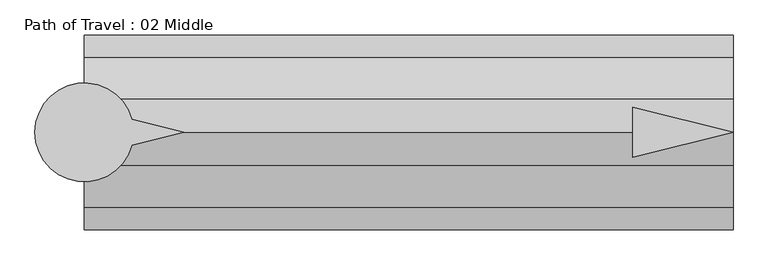
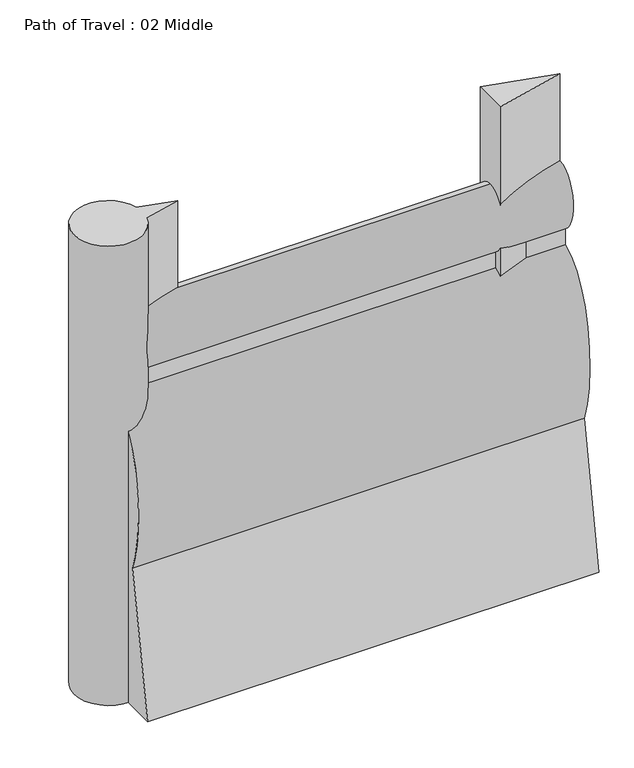
"""IFC4 building model written with IfcOpenShell, lengths in millimetres: proxy geometry, Path of Travel : 02 Middle."""

import ifcopenshell
import ifcopenshell.guid

model = None  # the IFC model being written
_history = None  # IfcOwnerHistory: only IFC2X3 demands one
_inside = {}  # id of a spatial element -> (the spatial element, [elements in it])
_under = {}  # id of a project, library or spatial element -> (it, [spatial elements below it])
_declared = {}  # id of a project -> (the project, [libraries it declares])
_typed = {}  # id of a type object -> (the type object, [elements of that type])
_made_of = {}  # id of a material, layer set ... -> (it, [elements and type objects made of it])


def new_model(schema):
    """Start an empty IFC model of exactly this schema.

    Asked for "IFC4X3", IfcOpenShell would pick the latest addendum, in which some entities
    have other attributes; the version numbers below select the first issue.
    IFC2X3 requires an IfcOwnerHistory on every rooted entity: one is made here for all.
    """
    global model, _history
    if schema == "IFC4X3":
        model = ifcopenshell.file(schema_version=(4, 3, 0, 0))
    else:
        model = ifcopenshell.file(schema=schema)
    _inside.clear()
    _under.clear()
    _declared.clear()
    _typed.clear()
    _made_of.clear()
    _history = None
    if model.schema == "IFC2X3":
        org = make("IfcOrganization", Name="unknown")
        user = make(
            "IfcPersonAndOrganization",
            ThePerson=make("IfcPerson", FamilyName="unknown"),
            TheOrganization=org,
        )
        app = make(
            "IfcApplication",
            ApplicationDeveloper=org,
            Version="unknown",
            ApplicationFullName="unknown",
            ApplicationIdentifier="unknown",
        )
        _history = make(
            "IfcOwnerHistory",
            OwningUser=user,
            OwningApplication=app,
            ChangeAction="ADDED",
            CreationDate=0,
        )
    return model


def make(cls, **values):
    """One entity of the class cls with the attributes given. An attribute that is None is left unset."""
    return model.create_entity(
        cls, **{name: value for name, value in values.items() if value is not None}
    )


def rooted(cls, **values):
    """An entity with a GlobalId (a new one), such as an element, a storey or a relation."""
    return make(cls, GlobalId=ifcopenshell.guid.new(), OwnerHistory=_history, **values)


def si_unit(unit_type, name, prefix=None):
    """IfcSIUnit, for example si_unit("LENGTHUNIT", "METRE", prefix="MILLI")."""
    return make("IfcSIUnit", UnitType=unit_type, Prefix=prefix, Name=name)


def assignment(units):
    """IfcUnitAssignment: the units of a project."""
    return None if units is None else make("IfcUnitAssignment", Units=units)


def point(xyz):
    """IfcCartesianPoint."""
    return None if xyz is None else make("IfcCartesianPoint", Coordinates=xyz)


def direction(xyz):
    """IfcDirection."""
    return None if xyz is None else make("IfcDirection", DirectionRatios=xyz)


def frame(location, z_axis=None, x_axis=None):
    """IfcAxis2Placement3D, a coordinate frame: its origin and axes. An axis left out is left unset."""
    return make(
        "IfcAxis2Placement3D",
        Location=point(location),
        Axis=direction(z_axis),
        RefDirection=direction(x_axis),
    )


def frame_2d(location, x_axis=None):
    """IfcAxis2Placement2D, a coordinate frame in the plane: its origin and x axis."""
    return make(
        "IfcAxis2Placement2D", Location=point(location), RefDirection=direction(x_axis)
    )


def origin():
    """The frame at (0, 0, 0) with its axes left unset."""
    return frame((0.0, 0.0, 0.0))


def origin_with_axes():
    """The frame at (0, 0, 0) with the z axis (0, 0, 1) and the x axis (1, 0, 0) written out."""
    return frame((0.0, 0.0, 0.0), z_axis=(0.0, 0.0, 1.0), x_axis=(1.0, 0.0, 0.0))


def place(relative_to, where):
    """IfcLocalPlacement: puts the frame where relative to a parent placement (None: the world)."""
    return make(
        "IfcLocalPlacement", PlacementRelTo=relative_to, RelativePlacement=where
    )


def context(
    kind, dimensions, precision=None, world=None, true_north=None, identifier=None
):
    """IfcGeometricRepresentationContext, for example the 3D "Model" context."""
    return make(
        "IfcGeometricRepresentationContext",
        ContextIdentifier=identifier,
        ContextType=kind,
        CoordinateSpaceDimension=dimensions,
        Precision=precision,
        WorldCoordinateSystem=world,
        TrueNorth=true_north,
    )


def project(units=None, contexts=None):
    """IfcProject with its units and contexts."""
    return rooted(
        "IfcProject",
        Name="project",
        RepresentationContexts=contexts,
        UnitsInContext=assignment(units),
    )


def spatial(cls, under=None, at=None, **own):
    """A site, building, storey or space (cls), placed at a placement, below another one or the project."""
    s = rooted(cls, ObjectPlacement=at, **own)
    if under is not None:
        _under.setdefault(under.id(), (under, []))[1].append(s)
    return s


def polyline(points):
    """IfcPolyline through the points."""
    return make("IfcPolyline", Points=[point(p) for p in points])


def circle_curve(where, radius):
    """IfcCircle in the frame where."""
    return make("IfcCircle", Position=where, Radius=radius)


def ellipse_curve(where, semi_axis1, semi_axis2):
    """IfcEllipse in the frame where."""
    return make(
        "IfcEllipse", Position=where, SemiAxis1=semi_axis1, SemiAxis2=semi_axis2
    )


def trimmed(basis, trim1, trim2, sense, master):
    """IfcTrimmedCurve: the piece of a basis curve between two trims."""
    return make(
        "IfcTrimmedCurve",
        BasisCurve=basis,
        Trim1=trim1,
        Trim2=trim2,
        SenseAgreement=sense,
        MasterRepresentation=master,
    )


def segment(curve, same_sense, transition):
    """IfcCompositeCurveSegment."""
    return make(
        "IfcCompositeCurveSegment",
        Transition=transition,
        SameSense=same_sense,
        ParentCurve=curve,
    )


def composite_curve(segments, self_intersect=None):
    """IfcCompositeCurve: segments joined end to end."""
    return make("IfcCompositeCurve", Segments=segments, SelfIntersect=self_intersect)


def outline(outer, holes=None, kind="AREA"):
    """IfcArbitraryClosedProfileDef: a profile drawn as a closed curve; with holes, ...WithVoids."""
    if holes is None:
        return make("IfcArbitraryClosedProfileDef", ProfileType=kind, OuterCurve=outer)
    return make(
        "IfcArbitraryProfileDefWithVoids",
        ProfileType=kind,
        OuterCurve=outer,
        InnerCurves=holes,
    )


def extrude(swept, where, along, depth):
    """IfcExtrudedAreaSolid: the profile swept, set in the frame where, extruded along a direction by depth."""
    return make(
        "IfcExtrudedAreaSolid",
        SweptArea=swept,
        Position=where,
        ExtrudedDirection=direction(along),
        Depth=depth,
    )


def shape(context_of_items, identifier, shape_type, items):
    """IfcShapeRepresentation: the items that make up one representation, for example the "Body"."""
    return make(
        "IfcShapeRepresentation",
        ContextOfItems=context_of_items,
        RepresentationIdentifier=identifier,
        RepresentationType=shape_type,
        Items=items,
    )


def source(mapping_origin, context_of_items, identifier, shape_type, items):
    """IfcRepresentationMap: a shape defined once, which mapped items show again and again."""
    return make(
        "IfcRepresentationMap",
        MappingOrigin=mapping_origin,
        MappedRepresentation=shape(context_of_items, identifier, shape_type, items),
    )


def transform(
    local_origin,
    x_axis=None,
    y_axis=None,
    z_axis=None,
    scale=None,
    scale2=None,
    scale3=None,
    uniform=True,
):
    """IfcCartesianTransformationOperator3D, or its non-uniform kind. x_axis, y_axis, z_axis: its Axis1, 2, 3."""
    if uniform:
        return make(
            "IfcCartesianTransformationOperator3D",
            Axis1=direction(x_axis),
            Axis2=direction(y_axis),
            LocalOrigin=point(local_origin),
            Scale=scale,
            Axis3=direction(z_axis),
        )
    return make(
        "IfcCartesianTransformationOperator3DnonUniform",
        Axis1=direction(x_axis),
        Axis2=direction(y_axis),
        LocalOrigin=point(local_origin),
        Scale=scale,
        Axis3=direction(z_axis),
        Scale2=scale2,
        Scale3=scale3,
    )


def mapped(mapping_source, mapping_target):
    """IfcMappedItem: shows the shape of a source again, moved by a transform."""
    return make(
        "IfcMappedItem", MappingSource=mapping_source, MappingTarget=mapping_target
    )


def made_of(thing, what):
    """Note that an element or type object is made of a material, layer set ...; save() writes the relation."""
    if what is not None:
        _made_of.setdefault(what.id(), (what, []))[1].append(thing)
    return thing


def element(
    cls,
    number,
    at=None,
    inside=None,
    cuts=None,
    type_object=None,
    material=None,
    context=None,
    identifier="Body",
    shape_type=None,
    held_by="IfcProductDefinitionShape",
    body=None,
    shapes=None,
    **own,
):
    """One element of the class cls, such as IfcWall. Its Tag is "e" and its number.

    at: its placement. inside: the storey or other place that contains it. cuts: it is an
    opening in that element (IfcRelVoidsElement). A single representation is given by context,
    identifier, shape_type and body (its items); several are given by shapes. held_by: the class
    of the entity that holds the representations. save() writes the other relations.
    """
    e = rooted(cls, Tag="e%d" % number, ObjectPlacement=at, **own)
    if body is not None:
        shapes = [shape(context, identifier, shape_type, body)]
    if shapes is not None:
        e.Representation = make(held_by, Representations=shapes)
    if inside is not None:
        _inside.setdefault(inside.id(), (inside, []))[1].append(e)
    if cuts is not None:
        rooted(
            "IfcRelVoidsElement", RelatingBuildingElement=cuts, RelatedOpeningElement=e
        )
    if type_object is not None:
        _typed.setdefault(type_object.id(), (type_object, []))[1].append(e)
    return made_of(e, material)


def aggregate(whole, parts):
    """IfcRelAggregates: a whole, such as a stair, and the parts it consists of."""
    return rooted("IfcRelAggregates", RelatingObject=whole, RelatedObjects=parts)


def save(model, path):
    """Write the relations noted so far, then the file.

    IfcRelAggregates (storeys below a building ...), IfcRelContainedInSpatialStructure (elements
    in a storey), IfcRelDefinesByType, IfcRelAssociatesMaterial and IfcRelDeclares: one each for
    every whole, place, type object, material and project.
    """
    for whole, parts in _under.values():
        aggregate(whole, parts)
    for where, things in _inside.values():
        rooted(
            "IfcRelContainedInSpatialStructure",
            RelatedElements=things,
            RelatingStructure=where,
        )
    for kind, things in _typed.values():
        rooted("IfcRelDefinesByType", RelatedObjects=things, RelatingType=kind)
    for what, things in _made_of.values():
        rooted("IfcRelAssociatesMaterial", RelatedObjects=things, RelatingMaterial=what)
    for by, libraries in _declared.values():
        rooted("IfcRelDeclares", RelatingContext=by, RelatedDefinitions=libraries)
    model.write(path)


def plane_surface(at):
    """IfcPlane: the flat surface through the origin of the frame at, square to its z axis."""
    return make("IfcPlane", Position=at)


def extruded_surface(curve, direction_of_extrusion, depth):
    """IfcSurfaceOfLinearExtrusion: the curve pushed along a direction by depth."""
    return make(
        "IfcSurfaceOfLinearExtrusion",
        SweptCurve=make("IfcArbitraryOpenProfileDef", ProfileType="CURVE", Curve=curve),
        ExtrudedDirection=direction(direction_of_extrusion),
        Depth=depth,
    )


def advanced_brep(points, edges, surfaces, faces):
    """IfcAdvancedBrep: a solid bounded by faces that lie on surfaces and meet in shared edges.

    An edge is (start, end): straight between two places in points (the first is 0);
    or (start, end, curve); or (start, end, curve, False) where it runs against its curve.
    A face is (place in surfaces, loops), or (place, loops, False) where it looks against
    its surface's normal. A loop lists edges by number (the first is 1), with a minus sign
    where the edge is run from its end to its start. The first loop is the outer one.
    """
    corners = [point(p) for p in points]
    vertices = [make("IfcVertexPoint", VertexGeometry=c) for c in corners]
    made = []
    for start, end, *more in edges:
        made.append(
            make(
                "IfcEdgeCurve",
                EdgeStart=vertices[start],
                EdgeEnd=vertices[end],
                EdgeGeometry=more[0] if more else make("IfcPolyline", Points=[corners[start], corners[end]]),
                SameSense=more[1] if len(more) > 1 else True,
            )
        )
    hull = []
    for where, loops, *sense in faces:
        bounds = []
        for j, loop in enumerate(loops):
            ring = [make("IfcOrientedEdge", EdgeElement=made[abs(k) - 1], Orientation=k > 0) for k in loop]
            bounds.append(
                make(
                    "IfcFaceOuterBound" if j == 0 else "IfcFaceBound",
                    Bound=make("IfcEdgeLoop", EdgeList=ring),
                    Orientation=True,
                )
            )
        hull.append(make("IfcAdvancedFace", Bounds=bounds, FaceSurface=surfaces[where], SameSense=sense[0] if sense else True))
    return make("IfcAdvancedBrep", Outer=make("IfcClosedShell", CfsFaces=hull))


def path_of_travel_02_middle_3236d784(model_context):
    return source(origin(), model_context, "Body", "SolidModel", [
        advanced_brep(
        [(227.5554837, 0.0, 1727.2), (227.5554837, 42.9018657, 1436.6534209), (227.5554837, 42.9018657, 1363.4763406), (227.5554837, 184.1186263, 643.4144547), (227.5554837, 297.5699544, 0.0), (227.5554837, 145.6574193, 0.0), (227.5554837, 0.0, 584.2), (227.5554837, -145.6574193, 0.0), (227.5554837, -297.5699544, 0.0), (227.5554837, -184.1186263, 643.4144547), (227.5554837, -42.9018657, 1363.4763406), (227.5554837, -42.9018657, 1436.6534209), (2208.7554837, 0.0, 1727.2), (2208.7554837, -42.9018657, 1436.6534209), (2208.7554837, -42.9018657, 1363.4763406), (2208.7554837, -184.1186263, 643.4144547), (2208.7554837, -297.5699544, 0.0), (2208.7554837, -145.6574193, 0.0), (2208.7554837, 0.0, 584.2), (2208.7554837, 145.6574193, 0.0), (2208.7554837, 297.5699544, 0.0), (2208.7554837, 184.1186263, 643.4144547), (2208.7554837, 42.9018657, 1363.4763406), (2208.7554837, 42.9018657, 1436.6534209)],
        [
            (0, 1, ellipse_curve(frame((227.5554837, 0.0, 1574.8), z_axis=(-1.0, 0.0, 0.0), x_axis=(0.0, 0.0, 1.0)), 152.4, 101.6)),
            (1, 2),
            (2, 3, ellipse_curve(frame((227.5554837, 0.0, 914.4), z_axis=(-1.0, 0.0, 0.0), x_axis=(0.0, 0.0, -1.0)), 457.2, 228.6)),
            (3, 4),
            (4, 5),
            (5, 6),
            (6, 7),
            (7, 8),
            (8, 9),
            (9, 10, ellipse_curve(frame((227.5554837, 0.0, 914.4), z_axis=(-1.0, 0.0, 0.0), x_axis=(0.0, 0.0, -1.0)), 457.2, 228.6)),
            (10, 11),
            (11, 0, ellipse_curve(frame((227.5554837, 0.0, 1574.8), z_axis=(-1.0, 0.0, 0.0), x_axis=(0.0, 0.0, 1.0)), 152.4, 101.6)),
            (12, 13, ellipse_curve(frame((2208.7554837, 0.0, 1574.8), z_axis=(1.0, 0.0, 0.0), x_axis=(0.0, 0.0, 1.0)), 152.4, 101.6)),
            (13, 14),
            (14, 15, ellipse_curve(frame((2208.7554837, 0.0, 914.4), z_axis=(1.0, 0.0, 0.0), x_axis=(0.0, 0.0, -1.0)), 457.2, 228.6)),
            (15, 16),
            (16, 17),
            (17, 18),
            (18, 19),
            (19, 20),
            (20, 21),
            (21, 22, ellipse_curve(frame((2208.7554837, 0.0, 914.4), z_axis=(1.0, 0.0, 0.0), x_axis=(0.0, 0.0, -1.0)), 457.2, 228.6)),
            (22, 23),
            (23, 12, ellipse_curve(frame((2208.7554837, 0.0, 1574.8), z_axis=(1.0, 0.0, 0.0), x_axis=(0.0, 0.0, 1.0)), 152.4, 101.6)),
            (0, 12),
            (23, 1),
            (22, 2),
            (21, 3),
            (20, 4),
            (19, 5),
            (18, 6),
            (17, 7),
            (16, 8),
            (15, 9),
            (14, 10),
            (13, 11),
        ],
        [
            plane_surface(frame((227.5554837, 0.0, 0.0), z_axis=(-1.0, 0.0, 0.0), x_axis=(0.0, 0.0, 1.0))),
            plane_surface(frame((2208.7554837, 0.0, 0.0), z_axis=(1.0, 0.0, 0.0), x_axis=(0.0, 0.0, 1.0))),
            extruded_surface(trimmed(ellipse_curve(frame((2208.7554837, 0.0, 1574.8), z_axis=(-1.0, 0.0, 0.0), x_axis=(0.0, 0.0, 1.0)), 152.4, 101.6), [point((2208.7554837, 0.0, 1727.2))], [point((2208.7554837, 42.9018657, 1436.6534209))], True, "CARTESIAN"), (-1981.1999999999998, 0.0, 0.0), 1981.1999999999998),
            plane_surface(frame((227.5554837, 42.9018657, 1436.6534209), z_axis=(0.0, 1.0, 0.0), x_axis=(1.0, 0.0, 0.0))),
            extruded_surface(trimmed(ellipse_curve(frame((2208.7554837, 0.0, 914.4), z_axis=(-1.0, 0.0, 0.0), x_axis=(0.0, 0.0, -1.0)), 457.2, 228.6), [point((2208.7554837, 42.9018657, 1363.4763406))], [point((2208.7554837, 184.1186263, 643.4144547))], True, "CARTESIAN"), (-1981.1999999999998, 0.0, 0.0), 1981.1999999999998),
            plane_surface(frame((227.5554837, 184.1186263, 643.4144547), z_axis=(0.0, 0.9848077530122078, 0.1736481776669322), x_axis=(1.0, 0.0, 0.0))),
            plane_surface(frame((227.5554837, 297.5699544, 0.0), z_axis=(0.0, 0.0, -1.0), x_axis=(1.0, 0.0, 0.0))),
            plane_surface(frame((227.5554837, 145.6574193, 0.0), z_axis=(0.0, -0.9702957262760199, -0.2419218955995739), x_axis=(1.0, 0.0, 0.0))),
            plane_surface(frame((227.5554837, 0.0, 584.2), z_axis=(0.0, 0.9702957262759961, -0.24192189559966923), x_axis=(1.0, 0.0, 0.0))),
            plane_surface(frame((227.5554837, -145.6574193, 0.0), z_axis=(0.0, 0.0, -1.0), x_axis=(1.0, 0.0, 0.0))),
            plane_surface(frame((227.5554837, -297.5699544, 0.0), z_axis=(0.0, -0.984807753012208, 0.17364817766693066), x_axis=(1.0, 0.0, 0.0))),
            extruded_surface(trimmed(ellipse_curve(frame((2208.7554837, 0.0, 914.4), z_axis=(-1.0, 0.0, 0.0), x_axis=(0.0, 0.0, -1.0)), 457.2, 228.6), [point((2208.7554837, -184.1186263, 643.4144547))], [point((2208.7554837, -42.9018657, 1363.4763406))], True, "CARTESIAN"), (-1981.1999999999998, 0.0, 0.0), 1981.1999999999998),
            plane_surface(frame((227.5554837, -42.9018657, 1363.4763406), z_axis=(0.0, -1.0, 0.0), x_axis=(1.0, 0.0, 0.0))),
            extruded_surface(trimmed(ellipse_curve(frame((2208.7554837, 0.0, 1574.8), z_axis=(-1.0, 0.0, 0.0), x_axis=(0.0, 0.0, 1.0)), 152.4, 101.6), [point((2208.7554837, -42.9018657, 1436.6534209))], [point((2208.7554837, 0.0, 1727.2))], True, "CARTESIAN"), (-1981.1999999999998, 0.0, 0.0), 1981.1999999999998),
        ],
        [
            (0, [[1, 2, 3, 4, 5, 6, 7, 8, 9, 10, 11, 12]]),
            (1, [[13, 14, 15, 16, 17, 18, 19, 20, 21, 22, 23, 24]]),
            (2, [[-1, 25, -24, 26]]),
            (3, [[-2, -26, -23, 27]]),
            (4, [[-3, -27, -22, 28]]),
            (5, [[-4, -28, -21, 29]]),
            (6, [[-5, -29, -20, 30]]),
            (7, [[-6, -30, -19, 31]]),
            (8, [[-7, -31, -18, 32]]),
            (9, [[-8, -32, -17, 33]]),
            (10, [[-9, -33, -16, 34]]),
            (11, [[-10, -34, -15, 35]]),
            (12, [[-11, -35, -14, 36]]),
            (13, [[-12, -36, -13, -25]]),
        ],
    ),
        extrude(outline(polyline([(1902.7503371, 76.2006338), (2208.7554837, 0.0), (1902.7503371, -76.2006338), (1902.7503371, 76.2006338)])), origin_with_axes(), (0.0, 0.0, 1.0), 2129.5973753),
        extrude(outline(composite_curve([segment(polyline([(372.7837828, 39.4440225), (531.182385, 0.0), (372.7837828, -39.4440225)]), True, "CONTINUOUS"), segment(trimmed(circle_curve(frame_2d((227.2200886, 0.0)), 150.8131956), [point((372.7837828, -39.4440225))], [point((372.7837828, 39.4440225))], False, "CARTESIAN"), True, "CONTINUOUS")], self_intersect=False)), origin_with_axes(), (0.0, 0.0, 1.0), 2129.5973753),
    ])


if __name__ == "__main__":
    model = new_model("IFC4")
    model_context = context("Model", 3, world=origin())
    ifc_project = project(units=[si_unit("LENGTHUNIT", "METRE", prefix="MILLI")], contexts=[model_context])
    site = spatial("IfcSite", under=ifc_project)
    building = spatial("IfcBuilding", under=site)
    placement = place(None, origin())
    path_of_travel_02_middle_shape = path_of_travel_02_middle_3236d784(model_context)
    element("IfcBuildingElementProxy", 1, Name="Path of Travel : 02 Middle", ObjectType="Path of Travel : 02 Middle", at=placement, inside=building, context=model_context, shape_type="MappedRepresentation", body=[
        mapped(path_of_travel_02_middle_shape, transform((0.0, 0.0, 0.0), x_axis=(1.0, 0.0, 0.0), y_axis=(0.0, 1.0, 0.0), z_axis=(0.0, 0.0, 1.0))),
    ])
    save(model, "model.ifc")

# Revit data of these elements
# Type "Path of Travel : 02 Middle"
#   Path of Egress [instance default] = 4' - 0"
#   built-in parameter 1001306 [instance default] = 4 (stored number, unit not read)
#   Dot at Start = no
#   Arrow in Middle = yes
#   Arrow at End = no
#   Egress Path = none
# Element 1 (IfcBuildingElementProxy, "Path of Travel : 02 Middle")
#   Path of Egress = 6' - 6"
#   built-in parameter 1001306 = 6.5 (stored number, unit not read)
#   Materials on its faces: "Egress Path Solid", "solid"
# Materials
#   "Egress Path Solid": class "Unassigned", colour RGB 255 128 64, transparency 0.75, Comments = "Rendering appearance not upgraded "
#   "solid": class "Generic", colour RGB 120 120 120, transparency 0, Cost = 0
